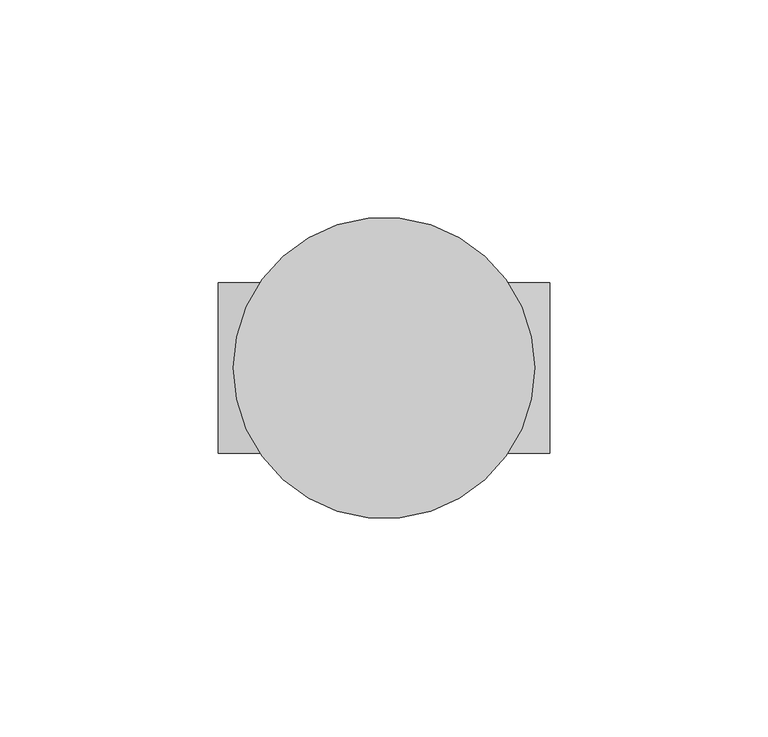
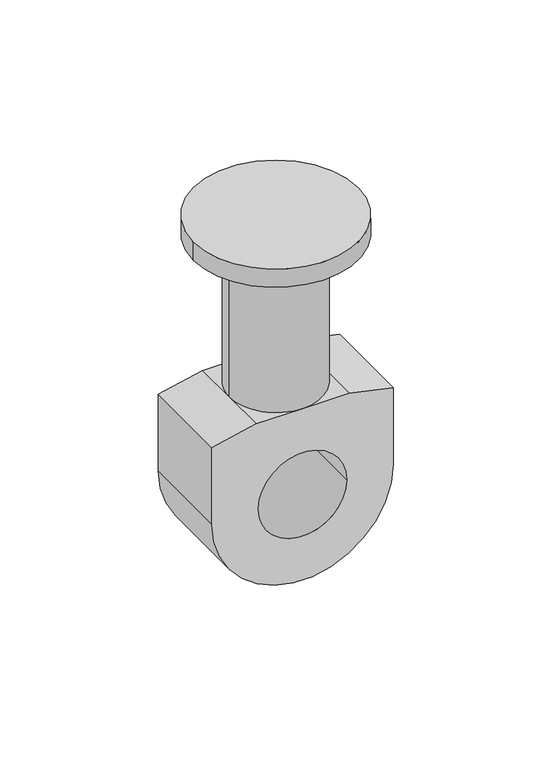
"""IFC4 building model written with IfcOpenShell, lengths in millimetres: fastener geometry, Spherical Head Eye Anchor : 6001-20.0-0250."""

import ifcopenshell
import ifcopenshell.guid

model = None  # the IFC model being written
_history = None  # IfcOwnerHistory: only IFC2X3 demands one
_inside = {}  # id of a spatial element -> (the spatial element, [elements in it])
_under = {}  # id of a project, library or spatial element -> (it, [spatial elements below it])
_declared = {}  # id of a project -> (the project, [libraries it declares])
_typed = {}  # id of a type object -> (the type object, [elements of that type])
_made_of = {}  # id of a material, layer set ... -> (it, [elements and type objects made of it])


def new_model(schema):
    """Start an empty IFC model of exactly this schema.

    Asked for "IFC4X3", IfcOpenShell would pick the latest addendum, in which some entities
    have other attributes; the version numbers below select the first issue.
    IFC2X3 requires an IfcOwnerHistory on every rooted entity: one is made here for all.
    """
    global model, _history
    if schema == "IFC4X3":
        model = ifcopenshell.file(schema_version=(4, 3, 0, 0))
    else:
        model = ifcopenshell.file(schema=schema)
    _inside.clear()
    _under.clear()
    _declared.clear()
    _typed.clear()
    _made_of.clear()
    _history = None
    if model.schema == "IFC2X3":
        org = make("IfcOrganization", Name="unknown")
        user = make(
            "IfcPersonAndOrganization",
            ThePerson=make("IfcPerson", FamilyName="unknown"),
            TheOrganization=org,
        )
        app = make(
            "IfcApplication",
            ApplicationDeveloper=org,
            Version="unknown",
            ApplicationFullName="unknown",
            ApplicationIdentifier="unknown",
        )
        _history = make(
            "IfcOwnerHistory",
            OwningUser=user,
            OwningApplication=app,
            ChangeAction="ADDED",
            CreationDate=0,
        )
    return model


def make(cls, **values):
    """One entity of the class cls with the attributes given. An attribute that is None is left unset."""
    return model.create_entity(
        cls, **{name: value for name, value in values.items() if value is not None}
    )


def rooted(cls, **values):
    """An entity with a GlobalId (a new one), such as an element, a storey or a relation."""
    return make(cls, GlobalId=ifcopenshell.guid.new(), OwnerHistory=_history, **values)


def si_unit(unit_type, name, prefix=None):
    """IfcSIUnit, for example si_unit("LENGTHUNIT", "METRE", prefix="MILLI")."""
    return make("IfcSIUnit", UnitType=unit_type, Prefix=prefix, Name=name)


def assignment(units):
    """IfcUnitAssignment: the units of a project."""
    return None if units is None else make("IfcUnitAssignment", Units=units)


def point(xyz):
    """IfcCartesianPoint."""
    return None if xyz is None else make("IfcCartesianPoint", Coordinates=xyz)


def direction(xyz):
    """IfcDirection."""
    return None if xyz is None else make("IfcDirection", DirectionRatios=xyz)


def frame(location, z_axis=None, x_axis=None):
    """IfcAxis2Placement3D, a coordinate frame: its origin and axes. An axis left out is left unset."""
    return make(
        "IfcAxis2Placement3D",
        Location=point(location),
        Axis=direction(z_axis),
        RefDirection=direction(x_axis),
    )


def origin():
    """The frame at (0, 0, 0) with its axes left unset."""
    return frame((0.0, 0.0, 0.0))


def place(relative_to, where):
    """IfcLocalPlacement: puts the frame where relative to a parent placement (None: the world)."""
    return make(
        "IfcLocalPlacement", PlacementRelTo=relative_to, RelativePlacement=where
    )


def context(
    kind, dimensions, precision=None, world=None, true_north=None, identifier=None
):
    """IfcGeometricRepresentationContext, for example the 3D "Model" context."""
    return make(
        "IfcGeometricRepresentationContext",
        ContextIdentifier=identifier,
        ContextType=kind,
        CoordinateSpaceDimension=dimensions,
        Precision=precision,
        WorldCoordinateSystem=world,
        TrueNorth=true_north,
    )


def project(units=None, contexts=None):
    """IfcProject with its units and contexts."""
    return rooted(
        "IfcProject",
        Name="project",
        RepresentationContexts=contexts,
        UnitsInContext=assignment(units),
    )


def spatial(cls, under=None, at=None, **own):
    """A site, building, storey or space (cls), placed at a placement, below another one or the project."""
    s = rooted(cls, ObjectPlacement=at, **own)
    if under is not None:
        _under.setdefault(under.id(), (under, []))[1].append(s)
    return s


def polyline(points):
    """IfcPolyline through the points."""
    return make("IfcPolyline", Points=[point(p) for p in points])


def circle_curve(where, radius):
    """IfcCircle in the frame where."""
    return make("IfcCircle", Position=where, Radius=radius)


def shape(context_of_items, identifier, shape_type, items):
    """IfcShapeRepresentation: the items that make up one representation, for example the "Body"."""
    return make(
        "IfcShapeRepresentation",
        ContextOfItems=context_of_items,
        RepresentationIdentifier=identifier,
        RepresentationType=shape_type,
        Items=items,
    )


def source(mapping_origin, context_of_items, identifier, shape_type, items):
    """IfcRepresentationMap: a shape defined once, which mapped items show again and again."""
    return make(
        "IfcRepresentationMap",
        MappingOrigin=mapping_origin,
        MappedRepresentation=shape(context_of_items, identifier, shape_type, items),
    )


def transform(
    local_origin,
    x_axis=None,
    y_axis=None,
    z_axis=None,
    scale=None,
    scale2=None,
    scale3=None,
    uniform=True,
):
    """IfcCartesianTransformationOperator3D, or its non-uniform kind. x_axis, y_axis, z_axis: its Axis1, 2, 3."""
    if uniform:
        return make(
            "IfcCartesianTransformationOperator3D",
            Axis1=direction(x_axis),
            Axis2=direction(y_axis),
            LocalOrigin=point(local_origin),
            Scale=scale,
            Axis3=direction(z_axis),
        )
    return make(
        "IfcCartesianTransformationOperator3DnonUniform",
        Axis1=direction(x_axis),
        Axis2=direction(y_axis),
        LocalOrigin=point(local_origin),
        Scale=scale,
        Axis3=direction(z_axis),
        Scale2=scale2,
        Scale3=scale3,
    )


def mapped(mapping_source, mapping_target):
    """IfcMappedItem: shows the shape of a source again, moved by a transform."""
    return make(
        "IfcMappedItem", MappingSource=mapping_source, MappingTarget=mapping_target
    )


def made_of(thing, what):
    """Note that an element or type object is made of a material, layer set ...; save() writes the relation."""
    if what is not None:
        _made_of.setdefault(what.id(), (what, []))[1].append(thing)
    return thing


def element(
    cls,
    number,
    at=None,
    inside=None,
    cuts=None,
    type_object=None,
    material=None,
    context=None,
    identifier="Body",
    shape_type=None,
    held_by="IfcProductDefinitionShape",
    body=None,
    shapes=None,
    **own,
):
    """One element of the class cls, such as IfcWall. Its Tag is "e" and its number.

    at: its placement. inside: the storey or other place that contains it. cuts: it is an
    opening in that element (IfcRelVoidsElement). A single representation is given by context,
    identifier, shape_type and body (its items); several are given by shapes. held_by: the class
    of the entity that holds the representations. save() writes the other relations.
    """
    e = rooted(cls, Tag="e%d" % number, ObjectPlacement=at, **own)
    if body is not None:
        shapes = [shape(context, identifier, shape_type, body)]
    if shapes is not None:
        e.Representation = make(held_by, Representations=shapes)
    if inside is not None:
        _inside.setdefault(inside.id(), (inside, []))[1].append(e)
    if cuts is not None:
        rooted(
            "IfcRelVoidsElement", RelatingBuildingElement=cuts, RelatedOpeningElement=e
        )
    if type_object is not None:
        _typed.setdefault(type_object.id(), (type_object, []))[1].append(e)
    return made_of(e, material)


def aggregate(whole, parts):
    """IfcRelAggregates: a whole, such as a stair, and the parts it consists of."""
    return rooted("IfcRelAggregates", RelatingObject=whole, RelatedObjects=parts)


def save(model, path):
    """Write the relations noted so far, then the file.

    IfcRelAggregates (storeys below a building ...), IfcRelContainedInSpatialStructure (elements
    in a storey), IfcRelDefinesByType, IfcRelAssociatesMaterial and IfcRelDeclares: one each for
    every whole, place, type object, material and project.
    """
    for whole, parts in _under.values():
        aggregate(whole, parts)
    for where, things in _inside.values():
        rooted(
            "IfcRelContainedInSpatialStructure",
            RelatedElements=things,
            RelatingStructure=where,
        )
    for kind, things in _typed.values():
        rooted("IfcRelDefinesByType", RelatedObjects=things, RelatingType=kind)
    for what, things in _made_of.values():
        rooted("IfcRelAssociatesMaterial", RelatedObjects=things, RelatingMaterial=what)
    for by, libraries in _declared.values():
        rooted("IfcRelDeclares", RelatingContext=by, RelatedDefinitions=libraries)
    model.write(path)


def plane_surface(at):
    """IfcPlane: the flat surface through the origin of the frame at, square to its z axis."""
    return make("IfcPlane", Position=at)


def cylinder_surface(at, radius):
    """IfcCylindricalSurface: all points at the distance radius from the z axis of the frame at."""
    return make("IfcCylindricalSurface", Position=at, Radius=radius)


def revolved_surface(curve, axis_point, axis_direction):
    """IfcSurfaceOfRevolution: the curve turned about the line through axis_point along axis_direction."""
    return make(
        "IfcSurfaceOfRevolution",
        SweptCurve=make("IfcArbitraryOpenProfileDef", ProfileType="CURVE", Curve=curve),
        AxisPosition=make("IfcAxis1Placement", Location=point(axis_point), Axis=direction(axis_direction)),
    )


def advanced_brep(points, edges, surfaces, faces):
    """IfcAdvancedBrep: a solid bounded by faces that lie on surfaces and meet in shared edges.

    An edge is (start, end): straight between two places in points (the first is 0);
    or (start, end, curve); or (start, end, curve, False) where it runs against its curve.
    A face is (place in surfaces, loops), or (place, loops, False) where it looks against
    its surface's normal. A loop lists edges by number (the first is 1), with a minus sign
    where the edge is run from its end to its start. The first loop is the outer one.
    """
    corners = [point(p) for p in points]
    vertices = [make("IfcVertexPoint", VertexGeometry=c) for c in corners]
    made = []
    for start, end, *more in edges:
        made.append(
            make(
                "IfcEdgeCurve",
                EdgeStart=vertices[start],
                EdgeEnd=vertices[end],
                EdgeGeometry=more[0] if more else make("IfcPolyline", Points=[corners[start], corners[end]]),
                SameSense=more[1] if len(more) > 1 else True,
            )
        )
    hull = []
    for where, loops, *sense in faces:
        bounds = []
        for j, loop in enumerate(loops):
            ring = [make("IfcOrientedEdge", EdgeElement=made[abs(k) - 1], Orientation=k > 0) for k in loop]
            bounds.append(
                make(
                    "IfcFaceOuterBound" if j == 0 else "IfcFaceBound",
                    Bound=make("IfcEdgeLoop", EdgeList=ring),
                    Orientation=True,
                )
            )
        hull.append(make("IfcAdvancedFace", Bounds=bounds, FaceSurface=surfaces[where], SameSense=sense[0] if sense else True))
    return make("IfcAdvancedBrep", Outer=make("IfcClosedShell", CfsFaces=hull))


def fastener_57157505(model_context):
    return source(origin(), model_context, "Body", "AdvancedBrep", [
        advanced_brep(
        [(-34.5, 0.0, -23.0), (34.5, 0.0, -23.0), (-19.5, 0.0, -23.0), (19.5, 0.0, -23.0), (34.5, 0.0, -15.0), (-34.5, 0.0, -15.0), (-38.0, -19.5, -127.0), (38.0, -19.5, -127.0), (38.0, -19.5, -93.0), (19.5, -19.5, -89.0), (0.0, -19.5, -89.0), (-19.5, -19.5, -89.0), (-38.0, -19.5, -93.0), (-18.5, -19.5, -127.0), (18.5, -19.5, -127.0), (38.0, 19.5, -127.0), (-38.0, 19.5, -127.0), (-38.0, 19.5, -93.0), (-19.5, 19.5, -89.0), (0.0, 19.5, -89.0), (19.5, 19.5, -89.0), (38.0, 19.5, -93.0), (18.5, 19.5, -127.0), (-18.5, 19.5, -127.0), (-19.5, 0.0, -89.0), (19.5, 0.0, -89.0)],
        [
            (0, 1, circle_curve(frame((0.0, 0.0, -23.0), z_axis=(0.0, 0.0, -1.0), x_axis=(1.0, 0.0, 0.0)), 34.5)),
            (1, 0, circle_curve(frame((0.0, 0.0, -23.0), z_axis=(0.0, 0.0, -1.0), x_axis=(1.0, 0.0, 0.0)), 34.5)),
            (2, 3, circle_curve(frame((0.0, 0.0, -23.0), z_axis=(0.0, 0.0, 1.0), x_axis=(1.0, 0.0, 0.0)), 19.5)),
            (3, 2, circle_curve(frame((0.0, 0.0, -23.0), z_axis=(0.0, 0.0, 1.0), x_axis=(1.0, 0.0, 0.0)), 19.5)),
            (4, 5, circle_curve(frame((0.0, 0.0, -15.0), z_axis=(0.0, 0.0, -1.0), x_axis=(1.0, 0.0, 0.0)), 34.5)),
            (5, 0),
            (1, 4),
            (5, 4, circle_curve(frame((0.0, 0.0, -15.0), z_axis=(0.0, 0.0, -1.0), x_axis=(1.0, 0.0, 0.0)), 34.5)),
            (6, 7, circle_curve(frame((0.0, -19.5, -127.0), z_axis=(0.0, -1.0, 0.0), x_axis=(-1.0, 0.0, 0.0)), 38.0)),
            (7, 8),
            (8, 9),
            (9, 10),
            (10, 11),
            (11, 12),
            (12, 6),
            (13, 14, circle_curve(frame((0.0, -19.5, -127.0), z_axis=(0.0, 1.0, 0.0), x_axis=(1.0, 0.0, 0.0)), 18.5)),
            (14, 13, circle_curve(frame((0.0, -19.5, -127.0), z_axis=(0.0, 1.0, 0.0), x_axis=(1.0, 0.0, 0.0)), 18.5)),
            (15, 16, circle_curve(frame((0.0, 19.5, -127.0), z_axis=(0.0, 1.0, 0.0), x_axis=(-1.0, 0.0, 0.0)), 38.0)),
            (16, 17),
            (17, 18),
            (18, 19),
            (19, 20),
            (20, 21),
            (21, 15),
            (22, 23, circle_curve(frame((0.0, 19.5, -127.0), z_axis=(0.0, -1.0, 0.0), x_axis=(1.0, 0.0, 0.0)), 18.5)),
            (23, 22, circle_curve(frame((0.0, 19.5, -127.0), z_axis=(0.0, -1.0, 0.0), x_axis=(1.0, 0.0, 0.0)), 18.5)),
            (17, 12),
            (11, 24),
            (24, 18),
            (9, 25),
            (25, 10, circle_curve(frame((0.0, 0.0, -89.0), z_axis=(0.0, 0.0, -1.0), x_axis=(1.0, 0.0, 0.0)), 19.5)),
            (10, 24, circle_curve(frame((0.0, 0.0, -89.0), z_axis=(0.0, 0.0, -1.0), x_axis=(1.0, 0.0, 0.0)), 19.5)),
            (24, 19, circle_curve(frame((0.0, 0.0, -89.0), z_axis=(0.0, 0.0, -1.0), x_axis=(1.0, 0.0, 0.0)), 19.5)),
            (19, 25, circle_curve(frame((0.0, 0.0, -89.0), z_axis=(0.0, 0.0, -1.0), x_axis=(1.0, 0.0, 0.0)), 19.5)),
            (25, 20),
            (8, 21),
            (7, 15),
            (16, 6),
            (22, 14),
            (13, 23),
            (25, 3),
            (2, 24),
        ],
        [
            plane_surface(frame((34.5, 0.0, -23.0), z_axis=(0.0, 0.0, -1.0), x_axis=(0.0, -1.0, 0.0))),
            cylinder_surface(frame((0.0, 0.0, -23.0), z_axis=(0.0, 0.0, 1.0), x_axis=(1.0, 0.0, 0.0)), 34.5),
            plane_surface(frame((-38.0, -19.5, -127.0), z_axis=(0.0, -1.0, 0.0), x_axis=(-1.0, 0.0, 0.0))),
            plane_surface(frame((-38.0, 19.5, -127.0), z_axis=(0.0, 1.0, 0.0), x_axis=(1.0, 0.0, 0.0))),
            plane_surface(frame((-38.0, 19.5, -93.0), z_axis=(-0.21133279252750878, 0.0, 0.9774141654398738), x_axis=(0.0, -1.0, 0.0))),
            plane_surface(frame((-19.5, 19.5, -89.0), z_axis=(0.0, 0.0, 1.0), x_axis=(0.0, -1.0, 0.0))),
            plane_surface(frame((19.5, 19.5, -89.0), z_axis=(0.2113327925273531, 0.0, 0.9774141654399074), x_axis=(0.0, -1.0, 0.0))),
            plane_surface(frame((38.0, 19.5, -93.0), z_axis=(1.0, 0.0, 0.0), x_axis=(0.0, -1.0, 0.0))),
            plane_surface(frame((-38.0, 19.5, -127.0), z_axis=(-1.0, 0.0, 0.0), x_axis=(0.0, -1.0, 0.0))),
            revolved_surface(polyline([(18.5, 19.5, -127.0), (18.5, -19.5, -127.0)]), (0.0, -19.5, -127.0), (0.0, 1.0, 0.0)),
            cylinder_surface(frame((0.0, 19.5, -127.0), z_axis=(0.0, -1.0, 0.0), x_axis=(-1.0, 0.0, 0.0)), 38.0),
            plane_surface(frame((19.5, 0.0, -15.0), z_axis=(0.0, 0.0, 1.0), x_axis=(0.0, 1.0, 0.0))),
            cylinder_surface(frame((0.0, 0.0, -127.0), z_axis=(0.0, 0.0, 1.0), x_axis=(1.0, 0.0, 0.0)), 19.5),
        ],
        [
            (0, [[1, 2], [3, 4]]),
            (1, [[5, 6, -2, 7]]),
            (1, [[8, -7, -1, -6]]),
            (2, [[9, 10, 11, 12, 13, 14, 15], [16, 17]]),
            (3, [[18, 19, 20, 21, 22, 23, 24], [25, 26]]),
            (4, [[-20, 27, -14, 28, 29]]),
            (5, [[-12, 30, 31]]),
            (5, [[-13, 32, -28]]),
            (5, [[-21, -29, 33]]),
            (5, [[-22, 34, 35]]),
            (6, [[-23, -35, -30, -11, 36]]),
            (7, [[-24, -36, -10, 37]]),
            (8, [[-19, 38, -15, -27]]),
            (9, [[39, -16, 40, -25]]),
            (9, [[-39, -26, -40, -17]]),
            (10, [[-9, -38, -18, -37]]),
            (11, [[-5, -8]]),
            (12, [[-31, 41, -3, 42, -32]]),
            (12, [[-33, -42, -4, -41, -34]]),
        ],
    ),
    ])


if __name__ == "__main__":
    model = new_model("IFC4")
    model_context = context("Model", 3, world=origin())
    ifc_project = project(units=[si_unit("LENGTHUNIT", "METRE", prefix="MILLI")], contexts=[model_context])
    site = spatial("IfcSite", under=ifc_project)
    building = spatial("IfcBuilding", under=site)
    placement = place(None, origin())
    fastener_shape = fastener_57157505(model_context)
    element("IfcFastener", 1, ObjectType="Spherical Head Eye Anchor : 6001-20.0-0250", at=placement, inside=building, context=model_context, shape_type="MappedRepresentation", body=[
        mapped(fastener_shape, transform((0.0, 0.0, 0.0), x_axis=(1.0, 0.0, 0.0), y_axis=(0.0, 1.0, 0.0), z_axis=(0.0, 0.0, 1.0))),
    ])
    save(model, "model.ifc")

# Revit data of these elements
# Type "Spherical Head Eye Anchor : 6001-20.0-0250"
#   Type Comments = "Mountingpart"
#   t2 = 4 mm
#   t1 = 8 mm
#   r3 = 18.5 mm
#   r2 = 38 mm
#   r1 = 34.5 mm
#   r = 19.5 mm
#   l = 150 mm
#   k = 15 mm
#   d2 = 76 mm
#   d1 = 69 mm
#   d = 39 mm
#   c = 37 mm
#   R = 80 mm
#   Da = 160 mm
#   Anchor Material [instance default] = Metal - Steel - S235
#   Default Elevation = 0
# Element 1 (IfcFastener, "Spherical Head Eye Anchor : 6001-20.0-0250")
#   Materials on its faces: "Metal - Steel - S235"
# Materials
#   "Metal - Steel - S235": class "Steel", colour RGB 247 247 247, transparency 0, Cost = 0
